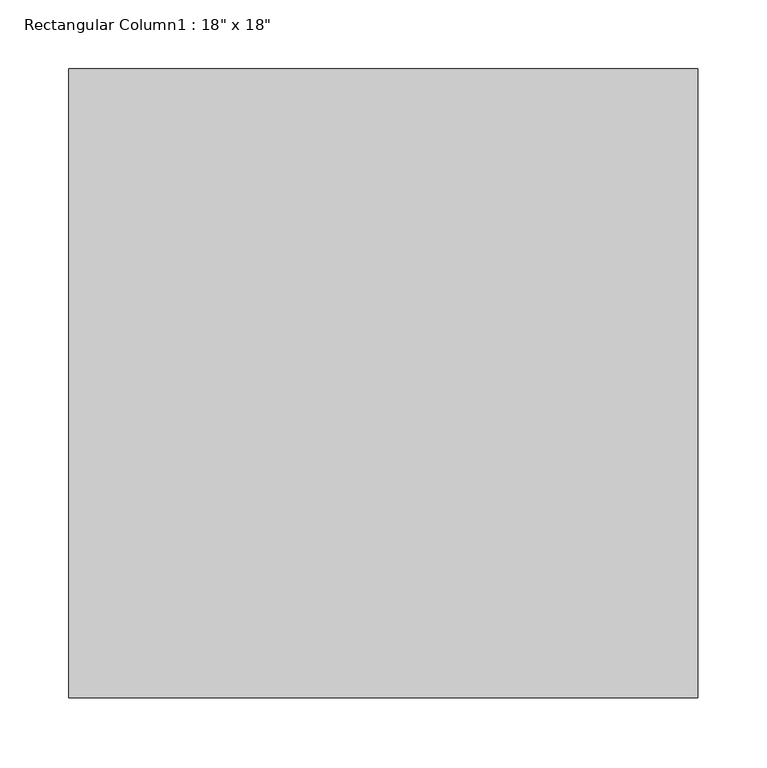
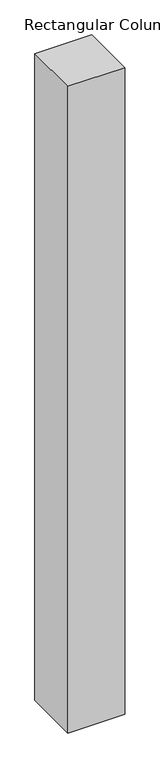
"""IFC4 building model written with IfcOpenShell, lengths in millimetres: column geometry."""

from ifc_helpers import new_model, si_unit, origin, origin_with_axes, place, context, project, spatial, polyline, outline, extrude, source, transform, mapped, element, save


def column_b6e10527(model_context):
    return source(origin(), model_context, "Body", "SweptSolid", [
        extrude(outline(polyline([(228.6, 228.6), (228.6, -228.6), (-228.6, -228.6), (-228.6, 228.6), (228.6, 228.6)])), origin_with_axes(), (0.0, 0.0, 1.0), 5486.4),
    ])


if __name__ == "__main__":
    model = new_model("IFC4")
    model_context = context("Model", 3, world=origin())
    ifc_project = project(units=[si_unit("LENGTHUNIT", "METRE", prefix="MILLI")], contexts=[model_context])
    site = spatial("IfcSite", under=ifc_project)
    building = spatial("IfcBuilding", under=site)
    placement = place(None, origin())
    column_shape = column_b6e10527(model_context)
    element("IfcColumn", 1, ObjectType="Rectangular Column1 : 18\" x 18\"", at=placement, inside=building, context=model_context, shape_type="MappedRepresentation", body=[
        mapped(column_shape, transform((0.0, 0.0, 0.0), x_axis=(1.0, 0.0, 0.0), y_axis=(0.0, 1.0, 0.0), z_axis=(0.0, 0.0, 1.0))),
    ])
    save(model, "model.ifc")

# Revit data of these elements
# Type "Rectangular Column1 : 18\" x 18\""
#   Depth = 1' - 6"
#   Width = 1' - 6"
